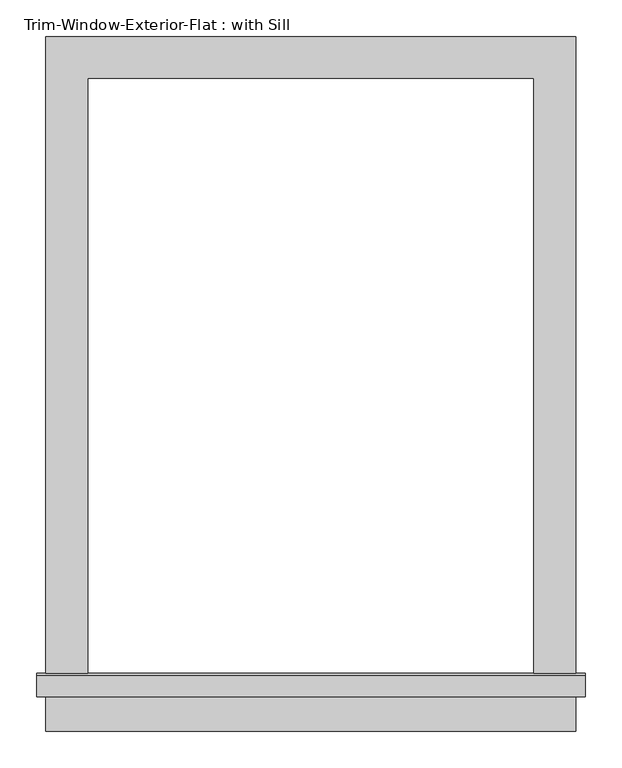
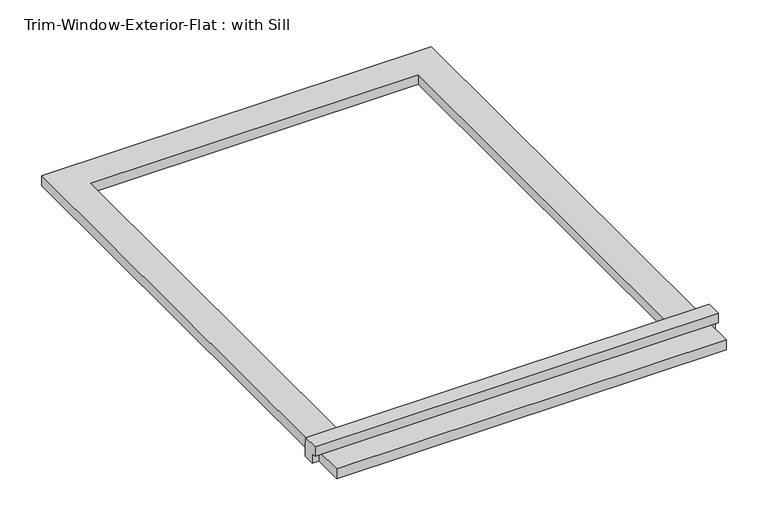
"""IFC4 building model written with IfcOpenShell, lengths in millimetres: proxy geometry, Trim-Window-Exterior-Flat : with Sill."""

from ifc_helpers import new_model, si_unit, frame, origin, origin_with_axes, place, context, project, spatial, polyline, outline, extrude, source, transform, mapped, element, save


def trim_window_exterior_flat_with_sill_a5919418(model_context):
    return source(origin(), model_context, "Body", "SweptSolid", [
        extrude(outline(polyline([(361.95, -834.9823709), (361.95, -892.1323709), (-361.95, -892.1323709), (-361.95, -834.9823709), (361.95, -834.9823709)])), origin_with_axes(), (0.0, 0.0, 1.0), 19.05),
        extrude(outline(polyline([(-844.55, 38.1), (-815.2580645, 38.1), (-812.8, 19.05), (-812.8, 0.0), (-834.9823709, 0.0), (-834.9823709, 19.05), (-844.55, 19.05), (-844.55, 38.1)])), frame((-374.65, 0.0, 0.0), z_axis=(1.0, 0.0, 0.0), x_axis=(0.0, 1.0, 0.0)), (0.0, 0.0, 1.0), 749.3),
        extrude(outline(polyline([(-361.95, 57.15), (361.95, 57.15), (361.95, -812.8), (304.8, -812.8), (304.8, 0.0), (-304.8, 0.0), (-304.8, -812.8), (-361.95, -812.8), (-361.95, 57.15)])), origin_with_axes(), (0.0, 0.0, 1.0), 19.05),
    ])


if __name__ == "__main__":
    model = new_model("IFC4")
    model_context = context("Model", 3, world=origin())
    ifc_project = project(units=[si_unit("LENGTHUNIT", "METRE", prefix="MILLI")], contexts=[model_context])
    site = spatial("IfcSite", under=ifc_project)
    building = spatial("IfcBuilding", under=site)
    placement = place(None, origin())
    trim_window_exterior_flat_with_sill_shape = trim_window_exterior_flat_with_sill_a5919418(model_context)
    element("IfcBuildingElementProxy", 1, Name="Trim-Window-Exterior-Flat : with Sill", ObjectType="Trim-Window-Exterior-Flat : with Sill", at=placement, inside=building, context=model_context, shape_type="MappedRepresentation", body=[
        mapped(trim_window_exterior_flat_with_sill_shape, transform((0.0, 0.0, 0.0), x_axis=(1.0, 0.0, 0.0), y_axis=(0.0, 1.0, 0.0), z_axis=(0.0, 0.0, 1.0))),
    ])
    save(model, "model.ifc")

# Revit data of these elements
# Type "Trim-Window-Exterior-Flat : with Sill"
#   Trim Width = 0' - 2 1/4"
#   Trim Thickness_Picture Frame = 0' - 1 1/4"
#   Trim Thickness_with Sill = 0' - 0 3/4"
#   Sill Thickness = 0' - 1 1/4"
#   Opening Width [instance default] = 2' - 0"
#   Opening Height [instance default] = 3' - 0"
#   Default Elevation = 4' - 0"
#   Sill = yes
#   Picture Frame = no
#   Trim Material [instance default] = none
# Element 1 (IfcBuildingElementProxy, "Trim-Window-Exterior-Flat : with Sill")
#   Opening Height = 2' - 8"
#   Trim Material = Clad - White
#   Materials on its faces: "Clad - White"
# Materials
#   "Clad - White": class "Wood", colour RGB 242 242 238, transparency 0, Cost = 0
